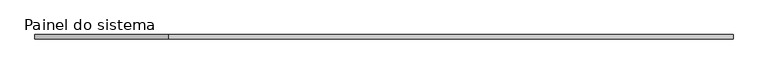
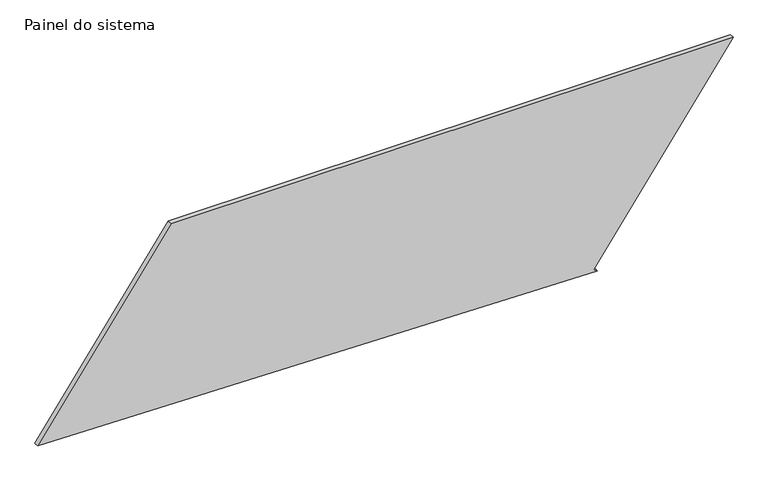
"""IFC4 building model written with IfcOpenShell, lengths in millimetres: plate geometry, Painel do sistema : Envidraçado."""

from ifc_helpers import new_model, si_unit, frame, origin, place, context, project, spatial, polyline, outline, extrude, source, transform, mapped, element, save


def painel_do_sistema_a2367732(model_context):
    return source(origin(), model_context, "Body", "SweptSolid", [
        extrude(outline(polyline([(0.0, 1177.8555446), (14.4529738, 1157.4567322), (1107.7563726, 1932.084444), (1107.7563726, -1190.1916239), (60.6547399, -1932.084444), (0.0, 1177.8555446)])), frame((0.0, 24.5, 0.0), z_axis=(0.0, 1.0, 0.0), x_axis=(0.0, 0.0, 1.0)), (0.0, 0.0, 1.0), 25.0),
    ])


if __name__ == "__main__":
    model = new_model("IFC4")
    model_context = context("Model", 3, world=origin())
    ifc_project = project(units=[si_unit("LENGTHUNIT", "METRE", prefix="MILLI")], contexts=[model_context])
    site = spatial("IfcSite", under=ifc_project)
    building = spatial("IfcBuilding", under=site)
    placement = place(None, origin())
    painel_do_sistema_shape = painel_do_sistema_a2367732(model_context)
    element("IfcPlate", 1, ObjectType="Painel do sistema : Envidraçado", at=placement, inside=building, context=model_context, shape_type="MappedRepresentation", body=[
        mapped(painel_do_sistema_shape, transform((0.0, 0.0, 0.0), x_axis=(1.0, 0.0, 0.0), y_axis=(0.0, 1.0, 0.0), z_axis=(0.0, 0.0, 1.0))),
    ])
    save(model, "model.ifc")

# Revit data of these elements
# Type "Painel do sistema : Envidraçado"
#   Construction Type Id = "GSP4R"
#   Analytic Construction = "Vidraça única Pilkington 1/8 pol"
#   Visual Light Transmittance = 0.9
#   Solar Heat Gain Coefficient = 0.86
#   Heat Transfer Coefficient (U) = 6.7069 W/(m²·K)
# Element 1 (IfcPlate, "Painel do sistema : Envidraçado")
#   Materials on its faces: "Vidro"
# Materials
#   "Vidro": class "Vidro", colour RGB 0 128 192, transparency 0.9, Description = "Vidro de sílica", Cost = 0
